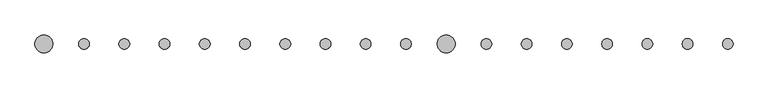
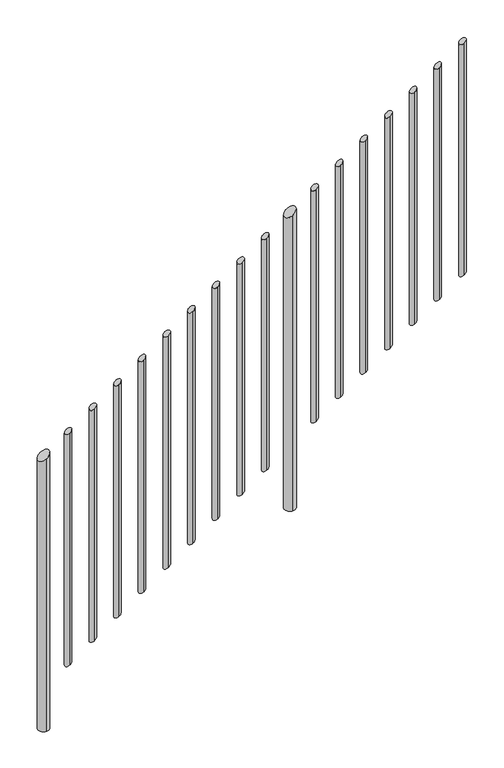
"""IFC4 building model written with IfcOpenShell, lengths in millimetres: railing geometry."""

from ifc_helpers import new_model, si_unit, frame, origin, place, context, project, spatial, circle_curve, ellipse_curve, source, transform, mapped, element, save
from ifc_brep_helpers import plane_surface, cylinder_surface, advanced_brep


def railing_d042ac98(model_context):
    return source(origin(), model_context, "Body", "AdvancedBrep", [
        advanced_brep(
        [(2380.725551, -1788.1965465, 2806.9021091), (2380.725551, -1788.1965465, 1868.75), (2380.725551, -1763.1965465, 1868.75), (2380.725551, -1763.1965465, 2806.9021091)],
        [
            (0, 1),
            (1, 2, ellipse_curve(frame((2380.725551, -1775.6965465, 1868.75), z_axis=(-0.5703958094953444, 0.0, 0.8213699656732956), x_axis=(0.8213699656732956, 0.0, 0.5703958094953445)), 15.2184771, 12.5)),
            (2, 3),
            (3, 0, ellipse_curve(frame((2380.725551, -1775.6965465, 2806.9021091), z_axis=(0.5703958094953457, 0.0, -0.8213699656732947), x_axis=(0.8213699656732947, 0.0, 0.5703958094953456)), 15.2184771, 12.5)),
            (0, 3, ellipse_curve(frame((2380.725551, -1775.6965465, 2806.9021091), z_axis=(0.5703958094953457, 0.0, -0.8213699656732947), x_axis=(0.8213699656732947, 0.0, 0.5703958094953456)), 15.2184771, 12.5)),
            (2, 1, ellipse_curve(frame((2380.725551, -1775.6965465, 1868.75), z_axis=(-0.5703958094953444, 0.0, 0.8213699656732956), x_axis=(0.8213699656732956, 0.0, 0.5703958094953445)), 15.2184771, 12.5)),
        ],
        [
            cylinder_surface(frame((2380.725551, -1775.6965465, 1768.75), z_axis=(0.0, 0.0, 1.0), x_axis=(0.0, 1.0, 0.0)), 12.5),
            plane_surface(frame((2405.725551, -1750.6965465, 2824.2632202), z_axis=(-0.5703958094953457, 0.0, 0.8213699656732947), x_axis=(0.0, -1.0, 0.0))),
            plane_surface(frame((2355.725551, -1750.6965465, 1851.3888889), z_axis=(0.5703958094953444, 0.0, -0.8213699656732956), x_axis=(0.0, -1.0, 0.0))),
        ],
        [
            (0, [[1, 2, 3, 4]]),
            (0, [[-1, 5, -3, 6]]),
            (1, [[-4, -5]]),
            (2, [[-2, -6]]),
        ],
    ),
        advanced_brep(
        [(2286.225551, -1788.1965465, 2741.2771091), (2286.225551, -1788.1965465, 1803.125), (2286.225551, -1763.1965465, 1803.125), (2286.225551, -1763.1965465, 2741.2771091)],
        [
            (0, 1),
            (1, 2, ellipse_curve(frame((2286.225551, -1775.6965465, 1803.125), z_axis=(-0.5703958094953444, 0.0, 0.8213699656732956), x_axis=(0.8213699656732956, 0.0, 0.5703958094953445)), 15.2184771, 12.5)),
            (2, 3),
            (3, 0, ellipse_curve(frame((2286.225551, -1775.6965465, 2741.2771091), z_axis=(0.5703958094953457, 0.0, -0.8213699656732947), x_axis=(0.8213699656732947, 0.0, 0.5703958094953456)), 15.2184771, 12.5)),
            (0, 3, ellipse_curve(frame((2286.225551, -1775.6965465, 2741.2771091), z_axis=(0.5703958094953457, 0.0, -0.8213699656732947), x_axis=(0.8213699656732947, 0.0, 0.5703958094953456)), 15.2184771, 12.5)),
            (2, 1, ellipse_curve(frame((2286.225551, -1775.6965465, 1803.125), z_axis=(-0.5703958094953444, 0.0, 0.8213699656732956), x_axis=(0.8213699656732956, 0.0, 0.5703958094953445)), 15.2184771, 12.5)),
        ],
        [
            cylinder_surface(frame((2286.225551, -1775.6965465, 1703.125), z_axis=(0.0, 0.0, 1.0), x_axis=(0.0, 1.0, 0.0)), 12.5),
            plane_surface(frame((2311.225551, -1750.6965465, 2758.6382202), z_axis=(-0.5703958094953457, 0.0, 0.8213699656732947), x_axis=(0.0, -1.0, 0.0))),
            plane_surface(frame((2261.225551, -1750.6965465, 1785.7638889), z_axis=(0.5703958094953444, 0.0, -0.8213699656732956), x_axis=(0.0, -1.0, 0.0))),
        ],
        [
            (0, [[1, 2, 3, 4]]),
            (0, [[-1, 5, -3, 6]]),
            (1, [[-4, -5]]),
            (2, [[-2, -6]]),
        ],
    ),
        advanced_brep(
        [(2191.725551, -1788.1965465, 2675.6521091), (2191.725551, -1788.1965465, 1737.5), (2191.725551, -1763.1965465, 1737.5), (2191.725551, -1763.1965465, 2675.6521091)],
        [
            (0, 1),
            (1, 2, ellipse_curve(frame((2191.725551, -1775.6965465, 1737.5), z_axis=(-0.5703958094953444, 0.0, 0.8213699656732956), x_axis=(0.8213699656732956, 0.0, 0.5703958094953445)), 15.2184771, 12.5)),
            (2, 3),
            (3, 0, ellipse_curve(frame((2191.725551, -1775.6965465, 2675.6521091), z_axis=(0.5703958094953457, 0.0, -0.8213699656732947), x_axis=(0.8213699656732947, 0.0, 0.5703958094953456)), 15.2184771, 12.5)),
            (0, 3, ellipse_curve(frame((2191.725551, -1775.6965465, 2675.6521091), z_axis=(0.5703958094953457, 0.0, -0.8213699656732947), x_axis=(0.8213699656732947, 0.0, 0.5703958094953456)), 15.2184771, 12.5)),
            (2, 1, ellipse_curve(frame((2191.725551, -1775.6965465, 1737.5), z_axis=(-0.5703958094953444, 0.0, 0.8213699656732956), x_axis=(0.8213699656732956, 0.0, 0.5703958094953445)), 15.2184771, 12.5)),
        ],
        [
            cylinder_surface(frame((2191.725551, -1775.6965465, 1637.5), z_axis=(0.0, 0.0, 1.0), x_axis=(0.0, 1.0, 0.0)), 12.5),
            plane_surface(frame((2216.725551, -1750.6965465, 2693.0132202), z_axis=(-0.5703958094953457, 0.0, 0.8213699656732947), x_axis=(0.0, -1.0, 0.0))),
            plane_surface(frame((2166.725551, -1750.6965465, 1720.1388889), z_axis=(0.5703958094953444, 0.0, -0.8213699656732956), x_axis=(0.0, -1.0, 0.0))),
        ],
        [
            (0, [[1, 2, 3, 4]]),
            (0, [[-1, 5, -3, 6]]),
            (1, [[-4, -5]]),
            (2, [[-2, -6]]),
        ],
    ),
        advanced_brep(
        [(2097.225551, -1788.1965465, 2610.0271091), (2097.225551, -1788.1965465, 1671.875), (2097.225551, -1763.1965465, 1671.875), (2097.225551, -1763.1965465, 2610.0271091)],
        [
            (0, 1),
            (1, 2, ellipse_curve(frame((2097.225551, -1775.6965465, 1671.875), z_axis=(-0.5703958094953444, 0.0, 0.8213699656732956), x_axis=(0.8213699656732956, 0.0, 0.5703958094953445)), 15.2184771, 12.5)),
            (2, 3),
            (3, 0, ellipse_curve(frame((2097.225551, -1775.6965465, 2610.0271091), z_axis=(0.5703958094953457, 0.0, -0.8213699656732947), x_axis=(0.8213699656732947, 0.0, 0.5703958094953456)), 15.2184771, 12.5)),
            (0, 3, ellipse_curve(frame((2097.225551, -1775.6965465, 2610.0271091), z_axis=(0.5703958094953457, 0.0, -0.8213699656732947), x_axis=(0.8213699656732947, 0.0, 0.5703958094953456)), 15.2184771, 12.5)),
            (2, 1, ellipse_curve(frame((2097.225551, -1775.6965465, 1671.875), z_axis=(-0.5703958094953444, 0.0, 0.8213699656732956), x_axis=(0.8213699656732956, 0.0, 0.5703958094953445)), 15.2184771, 12.5)),
        ],
        [
            cylinder_surface(frame((2097.225551, -1775.6965465, 1571.875), z_axis=(0.0, 0.0, 1.0), x_axis=(0.0, 1.0, 0.0)), 12.5),
            plane_surface(frame((2122.225551, -1750.6965465, 2627.3882202), z_axis=(-0.5703958094953457, 0.0, 0.8213699656732947), x_axis=(0.0, -1.0, 0.0))),
            plane_surface(frame((2072.225551, -1750.6965465, 1654.5138889), z_axis=(0.5703958094953444, 0.0, -0.8213699656732956), x_axis=(0.0, -1.0, 0.0))),
        ],
        [
            (0, [[1, 2, 3, 4]]),
            (0, [[-1, 5, -3, 6]]),
            (1, [[-4, -5]]),
            (2, [[-2, -6]]),
        ],
    ),
        advanced_brep(
        [(2002.725551, -1788.1965465, 2544.4021091), (2002.725551, -1788.1965465, 1606.25), (2002.725551, -1763.1965465, 1606.25), (2002.725551, -1763.1965465, 2544.4021091)],
        [
            (0, 1),
            (1, 2, ellipse_curve(frame((2002.725551, -1775.6965465, 1606.25), z_axis=(-0.5703958094953444, 0.0, 0.8213699656732956), x_axis=(0.8213699656732956, 0.0, 0.5703958094953445)), 15.2184771, 12.5)),
            (2, 3),
            (3, 0, ellipse_curve(frame((2002.725551, -1775.6965465, 2544.4021091), z_axis=(0.5703958094953457, 0.0, -0.8213699656732947), x_axis=(0.8213699656732947, 0.0, 0.5703958094953456)), 15.2184771, 12.5)),
            (0, 3, ellipse_curve(frame((2002.725551, -1775.6965465, 2544.4021091), z_axis=(0.5703958094953457, 0.0, -0.8213699656732947), x_axis=(0.8213699656732947, 0.0, 0.5703958094953456)), 15.2184771, 12.5)),
            (2, 1, ellipse_curve(frame((2002.725551, -1775.6965465, 1606.25), z_axis=(-0.5703958094953444, 0.0, 0.8213699656732956), x_axis=(0.8213699656732956, 0.0, 0.5703958094953445)), 15.2184771, 12.5)),
        ],
        [
            cylinder_surface(frame((2002.725551, -1775.6965465, 1506.25), z_axis=(0.0, 0.0, 1.0), x_axis=(0.0, 1.0, 0.0)), 12.5),
            plane_surface(frame((2027.725551, -1750.6965465, 2561.7632202), z_axis=(-0.5703958094953457, 0.0, 0.8213699656732947), x_axis=(0.0, -1.0, 0.0))),
            plane_surface(frame((1977.725551, -1750.6965465, 1588.8888889), z_axis=(0.5703958094953444, 0.0, -0.8213699656732956), x_axis=(0.0, -1.0, 0.0))),
        ],
        [
            (0, [[1, 2, 3, 4]]),
            (0, [[-1, 5, -3, 6]]),
            (1, [[-4, -5]]),
            (2, [[-2, -6]]),
        ],
    ),
        advanced_brep(
        [(1908.225551, -1788.1965465, 2478.7771091), (1908.225551, -1788.1965465, 1540.625), (1908.225551, -1763.1965465, 1540.625), (1908.225551, -1763.1965465, 2478.7771091)],
        [
            (0, 1),
            (1, 2, ellipse_curve(frame((1908.225551, -1775.6965465, 1540.625), z_axis=(-0.5703958094953444, 0.0, 0.8213699656732956), x_axis=(0.8213699656732956, 0.0, 0.5703958094953445)), 15.2184771, 12.5)),
            (2, 3),
            (3, 0, ellipse_curve(frame((1908.225551, -1775.6965465, 2478.7771091), z_axis=(0.5703958094953457, 0.0, -0.8213699656732947), x_axis=(0.8213699656732947, 0.0, 0.5703958094953456)), 15.2184771, 12.5)),
            (0, 3, ellipse_curve(frame((1908.225551, -1775.6965465, 2478.7771091), z_axis=(0.5703958094953457, 0.0, -0.8213699656732947), x_axis=(0.8213699656732947, 0.0, 0.5703958094953456)), 15.2184771, 12.5)),
            (2, 1, ellipse_curve(frame((1908.225551, -1775.6965465, 1540.625), z_axis=(-0.5703958094953444, 0.0, 0.8213699656732956), x_axis=(0.8213699656732956, 0.0, 0.5703958094953445)), 15.2184771, 12.5)),
        ],
        [
            cylinder_surface(frame((1908.225551, -1775.6965465, 1440.625), z_axis=(0.0, 0.0, 1.0), x_axis=(0.0, 1.0, 0.0)), 12.5),
            plane_surface(frame((1933.225551, -1750.6965465, 2496.1382202), z_axis=(-0.5703958094953457, 0.0, 0.8213699656732947), x_axis=(0.0, -1.0, 0.0))),
            plane_surface(frame((1883.225551, -1750.6965465, 1523.2638889), z_axis=(0.5703958094953444, 0.0, -0.8213699656732956), x_axis=(0.0, -1.0, 0.0))),
        ],
        [
            (0, [[1, 2, 3, 4]]),
            (0, [[-1, 5, -3, 6]]),
            (1, [[-4, -5]]),
            (2, [[-2, -6]]),
        ],
    ),
        advanced_brep(
        [(1813.725551, -1788.1965465, 2413.1521091), (1813.725551, -1788.1965465, 1475.0), (1813.725551, -1763.1965465, 1475.0), (1813.725551, -1763.1965465, 2413.1521091)],
        [
            (0, 1),
            (1, 2, ellipse_curve(frame((1813.725551, -1775.6965465, 1475.0), z_axis=(-0.5703958094953444, 0.0, 0.8213699656732956), x_axis=(0.8213699656732956, 0.0, 0.5703958094953445)), 15.2184771, 12.5)),
            (2, 3),
            (3, 0, ellipse_curve(frame((1813.725551, -1775.6965465, 2413.1521091), z_axis=(0.5703958094953457, 0.0, -0.8213699656732947), x_axis=(0.8213699656732947, 0.0, 0.5703958094953456)), 15.2184771, 12.5)),
            (0, 3, ellipse_curve(frame((1813.725551, -1775.6965465, 2413.1521091), z_axis=(0.5703958094953457, 0.0, -0.8213699656732947), x_axis=(0.8213699656732947, 0.0, 0.5703958094953456)), 15.2184771, 12.5)),
            (2, 1, ellipse_curve(frame((1813.725551, -1775.6965465, 1475.0), z_axis=(-0.5703958094953444, 0.0, 0.8213699656732956), x_axis=(0.8213699656732956, 0.0, 0.5703958094953445)), 15.2184771, 12.5)),
        ],
        [
            cylinder_surface(frame((1813.725551, -1775.6965465, 1375.0), z_axis=(0.0, 0.0, 1.0), x_axis=(0.0, 1.0, 0.0)), 12.5),
            plane_surface(frame((1838.725551, -1750.6965465, 2430.5132202), z_axis=(-0.5703958094953457, 0.0, 0.8213699656732947), x_axis=(0.0, -1.0, 0.0))),
            plane_surface(frame((1788.725551, -1750.6965465, 1457.6388889), z_axis=(0.5703958094953444, 0.0, -0.8213699656732956), x_axis=(0.0, -1.0, 0.0))),
        ],
        [
            (0, [[1, 2, 3, 4]]),
            (0, [[-1, 5, -3, 6]]),
            (1, [[-4, -5]]),
            (2, [[-2, -6]]),
        ],
    ),
        advanced_brep(
        [(1719.225551, -1796.6965465, 2347.5271091), (1719.225551, -1796.6965465, 1150.0), (1719.225551, -1754.6965465, 1150.0), (1719.225551, -1754.6965465, 2347.5271091)],
        [
            (0, 1),
            (1, 2, circle_curve(frame((1719.225551, -1775.6965465, 1150.0), z_axis=(0.0, 0.0, 1.0), x_axis=(0.0, 1.0, 0.0)), 21.0)),
            (2, 3),
            (3, 0, ellipse_curve(frame((1719.225551, -1775.6965465, 2347.5271091), z_axis=(0.5703958094953451, 0.0, -0.8213699656732952), x_axis=(0.8213699656732952, 0.0, 0.5703958094953447)), 25.5670415, 21.0)),
            (0, 3, ellipse_curve(frame((1719.225551, -1775.6965465, 2347.5271091), z_axis=(0.5703958094953451, 0.0, -0.8213699656732952), x_axis=(0.8213699656732952, 0.0, 0.5703958094953447)), 25.5670415, 21.0)),
            (2, 1, circle_curve(frame((1719.225551, -1775.6965465, 1150.0), z_axis=(0.0, 0.0, 1.0), x_axis=(0.0, 1.0, 0.0)), 21.0)),
        ],
        [
            cylinder_surface(frame((1719.225551, -1775.6965465, 1050.0), z_axis=(0.0, 0.0, 1.0), x_axis=(0.0, 1.0, 0.0)), 21.0),
            plane_surface(frame((1761.225551, -1733.6965465, 2376.6937758), z_axis=(-0.5703958094953451, 0.0, 0.8213699656732952), x_axis=(0.0, -1.0, 0.0))),
            plane_surface(frame((1677.225551, -1733.6965465, 1150.0), z_axis=(0.0, 0.0, -1.0), x_axis=(0.0, -1.0, 0.0))),
        ],
        [
            (0, [[1, 2, 3, 4]]),
            (0, [[-1, 5, -3, 6]]),
            (1, [[-4, -5]]),
            (2, [[-2, -6]]),
        ],
    ),
        advanced_brep(
        [(1624.725551, -1788.1965465, 2281.9021091), (1624.725551, -1788.1965465, 1343.75), (1624.725551, -1763.1965465, 1343.75), (1624.725551, -1763.1965465, 2281.9021091)],
        [
            (0, 1),
            (1, 2, ellipse_curve(frame((1624.725551, -1775.6965465, 1343.75), z_axis=(-0.5703958094953444, 0.0, 0.8213699656732956), x_axis=(0.8213699656732956, 0.0, 0.5703958094953445)), 15.2184771, 12.5)),
            (2, 3),
            (3, 0, ellipse_curve(frame((1624.725551, -1775.6965465, 2281.9021091), z_axis=(0.5703958094953457, 0.0, -0.8213699656732947), x_axis=(0.8213699656732947, 0.0, 0.5703958094953456)), 15.2184771, 12.5)),
            (0, 3, ellipse_curve(frame((1624.725551, -1775.6965465, 2281.9021091), z_axis=(0.5703958094953457, 0.0, -0.8213699656732947), x_axis=(0.8213699656732947, 0.0, 0.5703958094953456)), 15.2184771, 12.5)),
            (2, 1, ellipse_curve(frame((1624.725551, -1775.6965465, 1343.75), z_axis=(-0.5703958094953444, 0.0, 0.8213699656732956), x_axis=(0.8213699656732956, 0.0, 0.5703958094953445)), 15.2184771, 12.5)),
        ],
        [
            cylinder_surface(frame((1624.725551, -1775.6965465, 1243.75), z_axis=(0.0, 0.0, 1.0), x_axis=(0.0, 1.0, 0.0)), 12.5),
            plane_surface(frame((1649.725551, -1750.6965465, 2299.2632202), z_axis=(-0.5703958094953457, 0.0, 0.8213699656732947), x_axis=(0.0, -1.0, 0.0))),
            plane_surface(frame((1599.725551, -1750.6965465, 1326.3888889), z_axis=(0.5703958094953444, 0.0, -0.8213699656732956), x_axis=(0.0, -1.0, 0.0))),
        ],
        [
            (0, [[1, 2, 3, 4]]),
            (0, [[-1, 5, -3, 6]]),
            (1, [[-4, -5]]),
            (2, [[-2, -6]]),
        ],
    ),
        advanced_brep(
        [(1530.225551, -1788.1965465, 2216.2771091), (1530.225551, -1788.1965465, 1278.125), (1530.225551, -1763.1965465, 1278.125), (1530.225551, -1763.1965465, 2216.2771091)],
        [
            (0, 1),
            (1, 2, ellipse_curve(frame((1530.225551, -1775.6965465, 1278.125), z_axis=(-0.5703958094953444, 0.0, 0.8213699656732956), x_axis=(0.8213699656732956, 0.0, 0.5703958094953445)), 15.2184771, 12.5)),
            (2, 3),
            (3, 0, ellipse_curve(frame((1530.225551, -1775.6965465, 2216.2771091), z_axis=(0.5703958094953457, 0.0, -0.8213699656732947), x_axis=(0.8213699656732947, 0.0, 0.5703958094953456)), 15.2184771, 12.5)),
            (0, 3, ellipse_curve(frame((1530.225551, -1775.6965465, 2216.2771091), z_axis=(0.5703958094953457, 0.0, -0.8213699656732947), x_axis=(0.8213699656732947, 0.0, 0.5703958094953456)), 15.2184771, 12.5)),
            (2, 1, ellipse_curve(frame((1530.225551, -1775.6965465, 1278.125), z_axis=(-0.5703958094953444, 0.0, 0.8213699656732956), x_axis=(0.8213699656732956, 0.0, 0.5703958094953445)), 15.2184771, 12.5)),
        ],
        [
            cylinder_surface(frame((1530.225551, -1775.6965465, 1178.125), z_axis=(0.0, 0.0, 1.0), x_axis=(0.0, 1.0, 0.0)), 12.5),
            plane_surface(frame((1555.225551, -1750.6965465, 2233.6382202), z_axis=(-0.5703958094953457, 0.0, 0.8213699656732947), x_axis=(0.0, -1.0, 0.0))),
            plane_surface(frame((1505.225551, -1750.6965465, 1260.7638889), z_axis=(0.5703958094953444, 0.0, -0.8213699656732956), x_axis=(0.0, -1.0, 0.0))),
        ],
        [
            (0, [[1, 2, 3, 4]]),
            (0, [[-1, 5, -3, 6]]),
            (1, [[-4, -5]]),
            (2, [[-2, -6]]),
        ],
    ),
        advanced_brep(
        [(1435.725551, -1788.1965465, 2150.6521091), (1435.725551, -1788.1965465, 1212.5), (1435.725551, -1763.1965465, 1212.5), (1435.725551, -1763.1965465, 2150.6521091)],
        [
            (0, 1),
            (1, 2, ellipse_curve(frame((1435.725551, -1775.6965465, 1212.5), z_axis=(-0.5703958094953444, 0.0, 0.8213699656732956), x_axis=(0.8213699656732956, 0.0, 0.5703958094953445)), 15.2184771, 12.5)),
            (2, 3),
            (3, 0, ellipse_curve(frame((1435.725551, -1775.6965465, 2150.6521091), z_axis=(0.5703958094953457, 0.0, -0.8213699656732947), x_axis=(0.8213699656732947, 0.0, 0.5703958094953456)), 15.2184771, 12.5)),
            (0, 3, ellipse_curve(frame((1435.725551, -1775.6965465, 2150.6521091), z_axis=(0.5703958094953457, 0.0, -0.8213699656732947), x_axis=(0.8213699656732947, 0.0, 0.5703958094953456)), 15.2184771, 12.5)),
            (2, 1, ellipse_curve(frame((1435.725551, -1775.6965465, 1212.5), z_axis=(-0.5703958094953444, 0.0, 0.8213699656732956), x_axis=(0.8213699656732956, 0.0, 0.5703958094953445)), 15.2184771, 12.5)),
        ],
        [
            cylinder_surface(frame((1435.725551, -1775.6965465, 1112.5), z_axis=(0.0, 0.0, 1.0), x_axis=(0.0, 1.0, 0.0)), 12.5),
            plane_surface(frame((1460.725551, -1750.6965465, 2168.0132202), z_axis=(-0.5703958094953457, 0.0, 0.8213699656732947), x_axis=(0.0, -1.0, 0.0))),
            plane_surface(frame((1410.725551, -1750.6965465, 1195.1388889), z_axis=(0.5703958094953444, 0.0, -0.8213699656732956), x_axis=(0.0, -1.0, 0.0))),
        ],
        [
            (0, [[1, 2, 3, 4]]),
            (0, [[-1, 5, -3, 6]]),
            (1, [[-4, -5]]),
            (2, [[-2, -6]]),
        ],
    ),
        advanced_brep(
        [(1341.225551, -1788.1965465, 2085.0271091), (1341.225551, -1788.1965465, 1146.875), (1341.225551, -1763.1965465, 1146.875), (1341.225551, -1763.1965465, 2085.0271091)],
        [
            (0, 1),
            (1, 2, ellipse_curve(frame((1341.225551, -1775.6965465, 1146.875), z_axis=(-0.5703958094953444, 0.0, 0.8213699656732956), x_axis=(0.8213699656732956, 0.0, 0.5703958094953445)), 15.2184771, 12.5)),
            (2, 3),
            (3, 0, ellipse_curve(frame((1341.225551, -1775.6965465, 2085.0271091), z_axis=(0.5703958094953457, 0.0, -0.8213699656732947), x_axis=(0.8213699656732947, 0.0, 0.5703958094953456)), 15.2184771, 12.5)),
            (0, 3, ellipse_curve(frame((1341.225551, -1775.6965465, 2085.0271091), z_axis=(0.5703958094953457, 0.0, -0.8213699656732947), x_axis=(0.8213699656732947, 0.0, 0.5703958094953456)), 15.2184771, 12.5)),
            (2, 1, ellipse_curve(frame((1341.225551, -1775.6965465, 1146.875), z_axis=(-0.5703958094953444, 0.0, 0.8213699656732956), x_axis=(0.8213699656732956, 0.0, 0.5703958094953445)), 15.2184771, 12.5)),
        ],
        [
            cylinder_surface(frame((1341.225551, -1775.6965465, 1046.875), z_axis=(0.0, 0.0, 1.0), x_axis=(0.0, 1.0, 0.0)), 12.5),
            plane_surface(frame((1366.225551, -1750.6965465, 2102.3882202), z_axis=(-0.5703958094953457, 0.0, 0.8213699656732947), x_axis=(0.0, -1.0, 0.0))),
            plane_surface(frame((1316.225551, -1750.6965465, 1129.5138889), z_axis=(0.5703958094953444, 0.0, -0.8213699656732956), x_axis=(0.0, -1.0, 0.0))),
        ],
        [
            (0, [[1, 2, 3, 4]]),
            (0, [[-1, 5, -3, 6]]),
            (1, [[-4, -5]]),
            (2, [[-2, -6]]),
        ],
    ),
        advanced_brep(
        [(1246.725551, -1788.1965465, 2019.4021091), (1246.725551, -1788.1965465, 1081.25), (1246.725551, -1763.1965465, 1081.25), (1246.725551, -1763.1965465, 2019.4021091)],
        [
            (0, 1),
            (1, 2, ellipse_curve(frame((1246.725551, -1775.6965465, 1081.25), z_axis=(-0.5703958094953444, 0.0, 0.8213699656732956), x_axis=(0.8213699656732956, 0.0, 0.5703958094953445)), 15.2184771, 12.5)),
            (2, 3),
            (3, 0, ellipse_curve(frame((1246.725551, -1775.6965465, 2019.4021091), z_axis=(0.5703958094953457, 0.0, -0.8213699656732947), x_axis=(0.8213699656732947, 0.0, 0.5703958094953456)), 15.2184771, 12.5)),
            (0, 3, ellipse_curve(frame((1246.725551, -1775.6965465, 2019.4021091), z_axis=(0.5703958094953457, 0.0, -0.8213699656732947), x_axis=(0.8213699656732947, 0.0, 0.5703958094953456)), 15.2184771, 12.5)),
            (2, 1, ellipse_curve(frame((1246.725551, -1775.6965465, 1081.25), z_axis=(-0.5703958094953444, 0.0, 0.8213699656732956), x_axis=(0.8213699656732956, 0.0, 0.5703958094953445)), 15.2184771, 12.5)),
        ],
        [
            cylinder_surface(frame((1246.725551, -1775.6965465, 981.25), z_axis=(0.0, 0.0, 1.0), x_axis=(0.0, 1.0, 0.0)), 12.5),
            plane_surface(frame((1271.725551, -1750.6965465, 2036.7632202), z_axis=(-0.5703958094953457, 0.0, 0.8213699656732947), x_axis=(0.0, -1.0, 0.0))),
            plane_surface(frame((1221.725551, -1750.6965465, 1063.8888889), z_axis=(0.5703958094953444, 0.0, -0.8213699656732956), x_axis=(0.0, -1.0, 0.0))),
        ],
        [
            (0, [[1, 2, 3, 4]]),
            (0, [[-1, 5, -3, 6]]),
            (1, [[-4, -5]]),
            (2, [[-2, -6]]),
        ],
    ),
        advanced_brep(
        [(1152.225551, -1788.1965465, 1953.7771091), (1152.225551, -1788.1965465, 1015.625), (1152.225551, -1763.1965465, 1015.625), (1152.225551, -1763.1965465, 1953.7771091)],
        [
            (0, 1),
            (1, 2, ellipse_curve(frame((1152.225551, -1775.6965465, 1015.625), z_axis=(-0.5703958094953444, 0.0, 0.8213699656732956), x_axis=(0.8213699656732956, 0.0, 0.5703958094953445)), 15.2184771, 12.5)),
            (2, 3),
            (3, 0, ellipse_curve(frame((1152.225551, -1775.6965465, 1953.7771091), z_axis=(0.5703958094953457, 0.0, -0.8213699656732947), x_axis=(0.8213699656732947, 0.0, 0.5703958094953456)), 15.2184771, 12.5)),
            (0, 3, ellipse_curve(frame((1152.225551, -1775.6965465, 1953.7771091), z_axis=(0.5703958094953457, 0.0, -0.8213699656732947), x_axis=(0.8213699656732947, 0.0, 0.5703958094953456)), 15.2184771, 12.5)),
            (2, 1, ellipse_curve(frame((1152.225551, -1775.6965465, 1015.625), z_axis=(-0.5703958094953444, 0.0, 0.8213699656732956), x_axis=(0.8213699656732956, 0.0, 0.5703958094953445)), 15.2184771, 12.5)),
        ],
        [
            cylinder_surface(frame((1152.225551, -1775.6965465, 915.625), z_axis=(0.0, 0.0, 1.0), x_axis=(0.0, 1.0, 0.0)), 12.5),
            plane_surface(frame((1177.225551, -1750.6965465, 1971.1382202), z_axis=(-0.5703958094953457, 0.0, 0.8213699656732947), x_axis=(0.0, -1.0, 0.0))),
            plane_surface(frame((1127.225551, -1750.6965465, 998.2638889), z_axis=(0.5703958094953444, 0.0, -0.8213699656732956), x_axis=(0.0, -1.0, 0.0))),
        ],
        [
            (0, [[1, 2, 3, 4]]),
            (0, [[-1, 5, -3, 6]]),
            (1, [[-4, -5]]),
            (2, [[-2, -6]]),
        ],
    ),
        advanced_brep(
        [(1057.725551, -1788.1965465, 1888.1521091), (1057.725551, -1788.1965465, 950.0), (1057.725551, -1763.1965465, 950.0), (1057.725551, -1763.1965465, 1888.1521091)],
        [
            (0, 1),
            (1, 2, ellipse_curve(frame((1057.725551, -1775.6965465, 950.0), z_axis=(-0.5703958094953444, 0.0, 0.8213699656732956), x_axis=(0.8213699656732956, 0.0, 0.5703958094953445)), 15.2184771, 12.5)),
            (2, 3),
            (3, 0, ellipse_curve(frame((1057.725551, -1775.6965465, 1888.1521091), z_axis=(0.5703958094953457, 0.0, -0.8213699656732947), x_axis=(0.8213699656732947, 0.0, 0.5703958094953456)), 15.2184771, 12.5)),
            (0, 3, ellipse_curve(frame((1057.725551, -1775.6965465, 1888.1521091), z_axis=(0.5703958094953457, 0.0, -0.8213699656732947), x_axis=(0.8213699656732947, 0.0, 0.5703958094953456)), 15.2184771, 12.5)),
            (2, 1, ellipse_curve(frame((1057.725551, -1775.6965465, 950.0), z_axis=(-0.5703958094953444, 0.0, 0.8213699656732956), x_axis=(0.8213699656732956, 0.0, 0.5703958094953445)), 15.2184771, 12.5)),
        ],
        [
            cylinder_surface(frame((1057.725551, -1775.6965465, 850.0), z_axis=(0.0, 0.0, 1.0), x_axis=(0.0, 1.0, 0.0)), 12.5),
            plane_surface(frame((1082.725551, -1750.6965465, 1905.5132202), z_axis=(-0.5703958094953457, 0.0, 0.8213699656732947), x_axis=(0.0, -1.0, 0.0))),
            plane_surface(frame((1032.725551, -1750.6965465, 932.6388889), z_axis=(0.5703958094953444, 0.0, -0.8213699656732956), x_axis=(0.0, -1.0, 0.0))),
        ],
        [
            (0, [[1, 2, 3, 4]]),
            (0, [[-1, 5, -3, 6]]),
            (1, [[-4, -5]]),
            (2, [[-2, -6]]),
        ],
    ),
        advanced_brep(
        [(963.225551, -1788.1965465, 1822.5271091), (963.225551, -1788.1965465, 884.375), (963.225551, -1763.1965465, 884.375), (963.225551, -1763.1965465, 1822.5271091)],
        [
            (0, 1),
            (1, 2, ellipse_curve(frame((963.225551, -1775.6965465, 884.375), z_axis=(-0.5703958094953444, 0.0, 0.8213699656732956), x_axis=(0.8213699656732956, 0.0, 0.5703958094953445)), 15.2184771, 12.5)),
            (2, 3),
            (3, 0, ellipse_curve(frame((963.225551, -1775.6965465, 1822.5271091), z_axis=(0.5703958094953457, 0.0, -0.8213699656732947), x_axis=(0.8213699656732947, 0.0, 0.5703958094953456)), 15.2184771, 12.5)),
            (0, 3, ellipse_curve(frame((963.225551, -1775.6965465, 1822.5271091), z_axis=(0.5703958094953457, 0.0, -0.8213699656732947), x_axis=(0.8213699656732947, 0.0, 0.5703958094953456)), 15.2184771, 12.5)),
            (2, 1, ellipse_curve(frame((963.225551, -1775.6965465, 884.375), z_axis=(-0.5703958094953444, 0.0, 0.8213699656732956), x_axis=(0.8213699656732956, 0.0, 0.5703958094953445)), 15.2184771, 12.5)),
        ],
        [
            cylinder_surface(frame((963.225551, -1775.6965465, 784.375), z_axis=(0.0, 0.0, 1.0), x_axis=(0.0, 1.0, 0.0)), 12.5),
            plane_surface(frame((988.225551, -1750.6965465, 1839.8882202), z_axis=(-0.5703958094953457, 0.0, 0.8213699656732947), x_axis=(0.0, -1.0, 0.0))),
            plane_surface(frame((938.225551, -1750.6965465, 867.0138889), z_axis=(0.5703958094953444, 0.0, -0.8213699656732956), x_axis=(0.0, -1.0, 0.0))),
        ],
        [
            (0, [[1, 2, 3, 4]]),
            (0, [[-1, 5, -3, 6]]),
            (1, [[-4, -5]]),
            (2, [[-2, -6]]),
        ],
    ),
        advanced_brep(
        [(868.725551, -1788.1965465, 1756.9021091), (868.725551, -1788.1965465, 818.75), (868.725551, -1763.1965465, 818.75), (868.725551, -1763.1965465, 1756.9021091)],
        [
            (0, 1),
            (1, 2, ellipse_curve(frame((868.725551, -1775.6965465, 818.75), z_axis=(-0.5703958094953444, 0.0, 0.8213699656732956), x_axis=(0.8213699656732956, 0.0, 0.5703958094953445)), 15.2184771, 12.5)),
            (2, 3),
            (3, 0, ellipse_curve(frame((868.725551, -1775.6965465, 1756.9021091), z_axis=(0.5703958094953457, 0.0, -0.8213699656732947), x_axis=(0.8213699656732947, 0.0, 0.5703958094953456)), 15.2184771, 12.5)),
            (0, 3, ellipse_curve(frame((868.725551, -1775.6965465, 1756.9021091), z_axis=(0.5703958094953457, 0.0, -0.8213699656732947), x_axis=(0.8213699656732947, 0.0, 0.5703958094953456)), 15.2184771, 12.5)),
            (2, 1, ellipse_curve(frame((868.725551, -1775.6965465, 818.75), z_axis=(-0.5703958094953444, 0.0, 0.8213699656732956), x_axis=(0.8213699656732956, 0.0, 0.5703958094953445)), 15.2184771, 12.5)),
        ],
        [
            cylinder_surface(frame((868.725551, -1775.6965465, 718.75), z_axis=(0.0, 0.0, 1.0), x_axis=(0.0, 1.0, 0.0)), 12.5),
            plane_surface(frame((893.725551, -1750.6965465, 1774.2632202), z_axis=(-0.5703958094953457, 0.0, 0.8213699656732947), x_axis=(0.0, -1.0, 0.0))),
            plane_surface(frame((843.725551, -1750.6965465, 801.3888889), z_axis=(0.5703958094953444, 0.0, -0.8213699656732956), x_axis=(0.0, -1.0, 0.0))),
        ],
        [
            (0, [[1, 2, 3, 4]]),
            (0, [[-1, 5, -3, 6]]),
            (1, [[-4, -5]]),
            (2, [[-2, -6]]),
        ],
    ),
        advanced_brep(
        [(774.225551, -1796.6965465, 1691.2771091), (774.225551, -1796.6965465, 587.5), (774.225551, -1754.6965465, 587.5), (774.225551, -1754.6965465, 1691.2771091)],
        [
            (0, 1),
            (1, 2, circle_curve(frame((774.225551, -1775.6965465, 587.5), z_axis=(0.0, 0.0, 1.0), x_axis=(0.0, 1.0, 0.0)), 21.0)),
            (2, 3),
            (3, 0, ellipse_curve(frame((774.225551, -1775.6965465, 1691.2771091), z_axis=(0.5703958094953451, 0.0, -0.8213699656732952), x_axis=(0.8213699656732952, 0.0, 0.5703958094953447)), 25.5670415, 21.0)),
            (0, 3, ellipse_curve(frame((774.225551, -1775.6965465, 1691.2771091), z_axis=(0.5703958094953451, 0.0, -0.8213699656732952), x_axis=(0.8213699656732952, 0.0, 0.5703958094953447)), 25.5670415, 21.0)),
            (2, 1, circle_curve(frame((774.225551, -1775.6965465, 587.5), z_axis=(0.0, 0.0, 1.0), x_axis=(0.0, 1.0, 0.0)), 21.0)),
        ],
        [
            cylinder_surface(frame((774.225551, -1775.6965465, 487.5), z_axis=(0.0, 0.0, 1.0), x_axis=(0.0, 1.0, 0.0)), 21.0),
            plane_surface(frame((816.225551, -1733.6965465, 1720.4437758), z_axis=(-0.5703958094953451, 0.0, 0.8213699656732952), x_axis=(0.0, -1.0, 0.0))),
            plane_surface(frame((732.225551, -1733.6965465, 587.5), z_axis=(0.0, 0.0, -1.0), x_axis=(0.0, -1.0, 0.0))),
        ],
        [
            (0, [[1, 2, 3, 4]]),
            (0, [[-1, 5, -3, 6]]),
            (1, [[-4, -5]]),
            (2, [[-2, -6]]),
        ],
    ),
    ])


if __name__ == "__main__":
    model = new_model("IFC4")
    model_context = context("Model", 3, world=origin())
    ifc_project = project(units=[si_unit("LENGTHUNIT", "METRE", prefix="MILLI")], contexts=[model_context])
    site = spatial("IfcSite", under=ifc_project)
    building = spatial("IfcBuilding", under=site)
    placement = place(None, origin())
    railing_shape = railing_d042ac98(model_context)
    element("IfcRailing", 1, at=placement, inside=building, context=model_context, shape_type="MappedRepresentation", body=[
        mapped(railing_shape, transform((0.0, 0.0, 0.0), x_axis=(1.0, 0.0, 0.0), y_axis=(0.0, 1.0, 0.0), z_axis=(0.0, 0.0, 1.0))),
    ])
    save(model, "model.ifc")

# Revit data of these elements
# Element 1 (IfcRailing)
#   Materials on its faces: "Ferro - Pintura Esmalte"
# Materials
#   "Ferro - Pintura Esmalte": class "Pintura", colour RGB 255 255 255, transparency 0, Cost = 0
